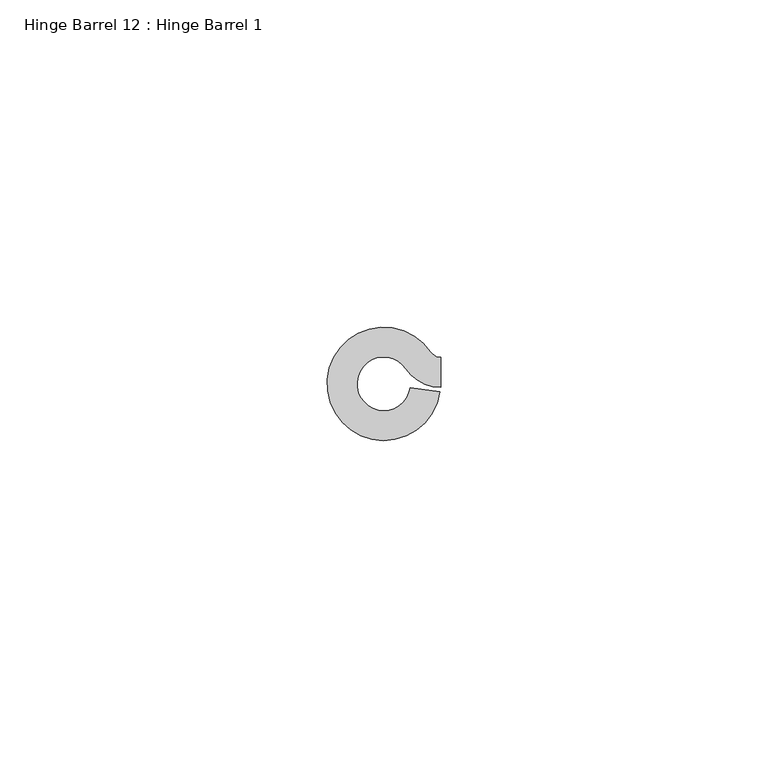
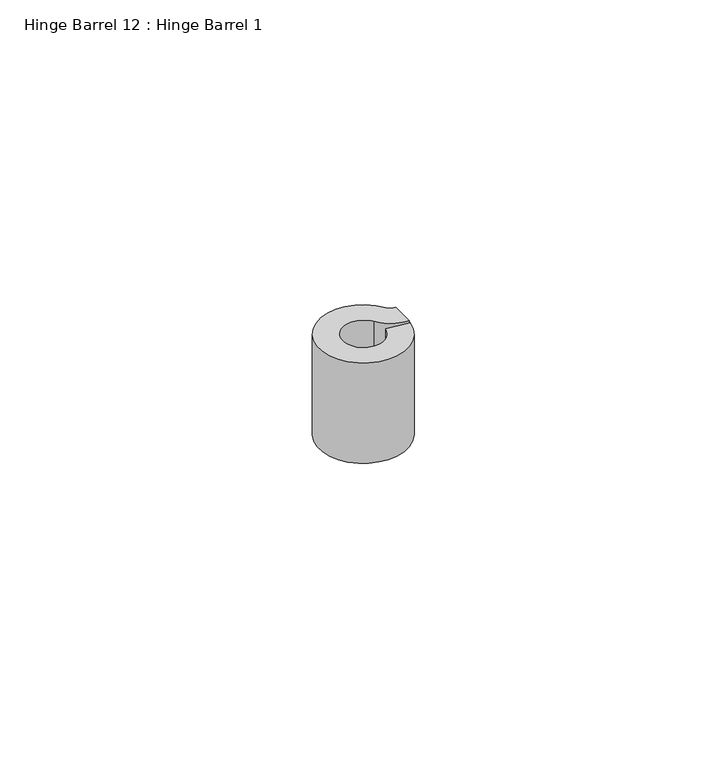
"""IFC4 building model written with IfcOpenShell, lengths in millimetres: proxy geometry, Hinge Barrel 12 : Hinge Barrel 1."""

import ifcopenshell
import ifcopenshell.guid

model = None  # the IFC model being written
_history = None  # IfcOwnerHistory: only IFC2X3 demands one
_inside = {}  # id of a spatial element -> (the spatial element, [elements in it])
_under = {}  # id of a project, library or spatial element -> (it, [spatial elements below it])
_declared = {}  # id of a project -> (the project, [libraries it declares])
_typed = {}  # id of a type object -> (the type object, [elements of that type])
_made_of = {}  # id of a material, layer set ... -> (it, [elements and type objects made of it])


def new_model(schema):
    """Start an empty IFC model of exactly this schema.

    Asked for "IFC4X3", IfcOpenShell would pick the latest addendum, in which some entities
    have other attributes; the version numbers below select the first issue.
    IFC2X3 requires an IfcOwnerHistory on every rooted entity: one is made here for all.
    """
    global model, _history
    if schema == "IFC4X3":
        model = ifcopenshell.file(schema_version=(4, 3, 0, 0))
    else:
        model = ifcopenshell.file(schema=schema)
    _inside.clear()
    _under.clear()
    _declared.clear()
    _typed.clear()
    _made_of.clear()
    _history = None
    if model.schema == "IFC2X3":
        org = make("IfcOrganization", Name="unknown")
        user = make(
            "IfcPersonAndOrganization",
            ThePerson=make("IfcPerson", FamilyName="unknown"),
            TheOrganization=org,
        )
        app = make(
            "IfcApplication",
            ApplicationDeveloper=org,
            Version="unknown",
            ApplicationFullName="unknown",
            ApplicationIdentifier="unknown",
        )
        _history = make(
            "IfcOwnerHistory",
            OwningUser=user,
            OwningApplication=app,
            ChangeAction="ADDED",
            CreationDate=0,
        )
    return model


def make(cls, **values):
    """One entity of the class cls with the attributes given. An attribute that is None is left unset."""
    return model.create_entity(
        cls, **{name: value for name, value in values.items() if value is not None}
    )


def rooted(cls, **values):
    """An entity with a GlobalId (a new one), such as an element, a storey or a relation."""
    return make(cls, GlobalId=ifcopenshell.guid.new(), OwnerHistory=_history, **values)


def si_unit(unit_type, name, prefix=None):
    """IfcSIUnit, for example si_unit("LENGTHUNIT", "METRE", prefix="MILLI")."""
    return make("IfcSIUnit", UnitType=unit_type, Prefix=prefix, Name=name)


def assignment(units):
    """IfcUnitAssignment: the units of a project."""
    return None if units is None else make("IfcUnitAssignment", Units=units)


def point(xyz):
    """IfcCartesianPoint."""
    return None if xyz is None else make("IfcCartesianPoint", Coordinates=xyz)


def direction(xyz):
    """IfcDirection."""
    return None if xyz is None else make("IfcDirection", DirectionRatios=xyz)


def frame(location, z_axis=None, x_axis=None):
    """IfcAxis2Placement3D, a coordinate frame: its origin and axes. An axis left out is left unset."""
    return make(
        "IfcAxis2Placement3D",
        Location=point(location),
        Axis=direction(z_axis),
        RefDirection=direction(x_axis),
    )


def frame_2d(location, x_axis=None):
    """IfcAxis2Placement2D, a coordinate frame in the plane: its origin and x axis."""
    return make(
        "IfcAxis2Placement2D", Location=point(location), RefDirection=direction(x_axis)
    )


def origin():
    """The frame at (0, 0, 0) with its axes left unset."""
    return frame((0.0, 0.0, 0.0))


def place(relative_to, where):
    """IfcLocalPlacement: puts the frame where relative to a parent placement (None: the world)."""
    return make(
        "IfcLocalPlacement", PlacementRelTo=relative_to, RelativePlacement=where
    )


def context(
    kind, dimensions, precision=None, world=None, true_north=None, identifier=None
):
    """IfcGeometricRepresentationContext, for example the 3D "Model" context."""
    return make(
        "IfcGeometricRepresentationContext",
        ContextIdentifier=identifier,
        ContextType=kind,
        CoordinateSpaceDimension=dimensions,
        Precision=precision,
        WorldCoordinateSystem=world,
        TrueNorth=true_north,
    )


def project(units=None, contexts=None):
    """IfcProject with its units and contexts."""
    return rooted(
        "IfcProject",
        Name="project",
        RepresentationContexts=contexts,
        UnitsInContext=assignment(units),
    )


def spatial(cls, under=None, at=None, **own):
    """A site, building, storey or space (cls), placed at a placement, below another one or the project."""
    s = rooted(cls, ObjectPlacement=at, **own)
    if under is not None:
        _under.setdefault(under.id(), (under, []))[1].append(s)
    return s


def polyline(points):
    """IfcPolyline through the points."""
    return make("IfcPolyline", Points=[point(p) for p in points])


def circle_curve(where, radius):
    """IfcCircle in the frame where."""
    return make("IfcCircle", Position=where, Radius=radius)


def trimmed(basis, trim1, trim2, sense, master):
    """IfcTrimmedCurve: the piece of a basis curve between two trims."""
    return make(
        "IfcTrimmedCurve",
        BasisCurve=basis,
        Trim1=trim1,
        Trim2=trim2,
        SenseAgreement=sense,
        MasterRepresentation=master,
    )


def segment(curve, same_sense, transition):
    """IfcCompositeCurveSegment."""
    return make(
        "IfcCompositeCurveSegment",
        Transition=transition,
        SameSense=same_sense,
        ParentCurve=curve,
    )


def composite_curve(segments, self_intersect=None):
    """IfcCompositeCurve: segments joined end to end."""
    return make("IfcCompositeCurve", Segments=segments, SelfIntersect=self_intersect)


def outline(outer, holes=None, kind="AREA"):
    """IfcArbitraryClosedProfileDef: a profile drawn as a closed curve; with holes, ...WithVoids."""
    if holes is None:
        return make("IfcArbitraryClosedProfileDef", ProfileType=kind, OuterCurve=outer)
    return make(
        "IfcArbitraryProfileDefWithVoids",
        ProfileType=kind,
        OuterCurve=outer,
        InnerCurves=holes,
    )


def extrude(swept, where, along, depth):
    """IfcExtrudedAreaSolid: the profile swept, set in the frame where, extruded along a direction by depth."""
    return make(
        "IfcExtrudedAreaSolid",
        SweptArea=swept,
        Position=where,
        ExtrudedDirection=direction(along),
        Depth=depth,
    )


def shape(context_of_items, identifier, shape_type, items):
    """IfcShapeRepresentation: the items that make up one representation, for example the "Body"."""
    return make(
        "IfcShapeRepresentation",
        ContextOfItems=context_of_items,
        RepresentationIdentifier=identifier,
        RepresentationType=shape_type,
        Items=items,
    )


def source(mapping_origin, context_of_items, identifier, shape_type, items):
    """IfcRepresentationMap: a shape defined once, which mapped items show again and again."""
    return make(
        "IfcRepresentationMap",
        MappingOrigin=mapping_origin,
        MappedRepresentation=shape(context_of_items, identifier, shape_type, items),
    )


def transform(
    local_origin,
    x_axis=None,
    y_axis=None,
    z_axis=None,
    scale=None,
    scale2=None,
    scale3=None,
    uniform=True,
):
    """IfcCartesianTransformationOperator3D, or its non-uniform kind. x_axis, y_axis, z_axis: its Axis1, 2, 3."""
    if uniform:
        return make(
            "IfcCartesianTransformationOperator3D",
            Axis1=direction(x_axis),
            Axis2=direction(y_axis),
            LocalOrigin=point(local_origin),
            Scale=scale,
            Axis3=direction(z_axis),
        )
    return make(
        "IfcCartesianTransformationOperator3DnonUniform",
        Axis1=direction(x_axis),
        Axis2=direction(y_axis),
        LocalOrigin=point(local_origin),
        Scale=scale,
        Axis3=direction(z_axis),
        Scale2=scale2,
        Scale3=scale3,
    )


def mapped(mapping_source, mapping_target):
    """IfcMappedItem: shows the shape of a source again, moved by a transform."""
    return make(
        "IfcMappedItem", MappingSource=mapping_source, MappingTarget=mapping_target
    )


def made_of(thing, what):
    """Note that an element or type object is made of a material, layer set ...; save() writes the relation."""
    if what is not None:
        _made_of.setdefault(what.id(), (what, []))[1].append(thing)
    return thing


def element(
    cls,
    number,
    at=None,
    inside=None,
    cuts=None,
    type_object=None,
    material=None,
    context=None,
    identifier="Body",
    shape_type=None,
    held_by="IfcProductDefinitionShape",
    body=None,
    shapes=None,
    **own,
):
    """One element of the class cls, such as IfcWall. Its Tag is "e" and its number.

    at: its placement. inside: the storey or other place that contains it. cuts: it is an
    opening in that element (IfcRelVoidsElement). A single representation is given by context,
    identifier, shape_type and body (its items); several are given by shapes. held_by: the class
    of the entity that holds the representations. save() writes the other relations.
    """
    e = rooted(cls, Tag="e%d" % number, ObjectPlacement=at, **own)
    if body is not None:
        shapes = [shape(context, identifier, shape_type, body)]
    if shapes is not None:
        e.Representation = make(held_by, Representations=shapes)
    if inside is not None:
        _inside.setdefault(inside.id(), (inside, []))[1].append(e)
    if cuts is not None:
        rooted(
            "IfcRelVoidsElement", RelatingBuildingElement=cuts, RelatedOpeningElement=e
        )
    if type_object is not None:
        _typed.setdefault(type_object.id(), (type_object, []))[1].append(e)
    return made_of(e, material)


def aggregate(whole, parts):
    """IfcRelAggregates: a whole, such as a stair, and the parts it consists of."""
    return rooted("IfcRelAggregates", RelatingObject=whole, RelatedObjects=parts)


def save(model, path):
    """Write the relations noted so far, then the file.

    IfcRelAggregates (storeys below a building ...), IfcRelContainedInSpatialStructure (elements
    in a storey), IfcRelDefinesByType, IfcRelAssociatesMaterial and IfcRelDeclares: one each for
    every whole, place, type object, material and project.
    """
    for whole, parts in _under.values():
        aggregate(whole, parts)
    for where, things in _inside.values():
        rooted(
            "IfcRelContainedInSpatialStructure",
            RelatedElements=things,
            RelatingStructure=where,
        )
    for kind, things in _typed.values():
        rooted("IfcRelDefinesByType", RelatedObjects=things, RelatingType=kind)
    for what, things in _made_of.values():
        rooted("IfcRelAssociatesMaterial", RelatedObjects=things, RelatingMaterial=what)
    for by, libraries in _declared.values():
        rooted("IfcRelDeclares", RelatingContext=by, RelatedDefinitions=libraries)
    model.write(path)


def hinge_barrel_12_hinge_barrel_1_babfa127(model_context):
    return source(origin(), model_context, "Body", "SweptSolid", [
        extrude(outline(composite_curve([segment(trimmed(circle_curve(frame_2d((587319.1320739, -531776.6049841)), 4.0894), [point((587322.5194669, -531774.3139665))], [point((587323.1821338, -531777.1708529))], True, "CARTESIAN"), True, "CONTINUOUS"), segment(polyline([(587323.1821338, -531777.1708529), (587327.7022899, -531777.8024028)]), True, "CONTINUOUS"), segment(trimmed(circle_curve(frame_2d((587319.1320739, -531776.6049841)), 8.6534625), [point((587327.7022899, -531777.8024028))], [point((587326.3000393, -531771.7570273))], False, "CARTESIAN"), True, "CONTINUOUS"), segment(trimmed(circle_curve(frame_2d((587327.8245257, -531770.7259615)), 1.8404226), [point((587326.3000393, -531771.7570273))], [point((587327.8245257, -531772.5663841))], True, "CARTESIAN"), True, "CONTINUOUS"), segment(polyline([(587327.8245257, -531772.5663841), (587327.8245257, -531777.1304466)]), True, "CONTINUOUS"), segment(trimmed(circle_curve(frame_2d((587327.8245257, -531770.7259615)), 6.4044851), [point((587327.8245257, -531777.1304466))], [point((587322.5194669, -531774.3139665))], False, "CARTESIAN"), True, "CONTINUOUS")], self_intersect=False)), frame((0.0, 0.0, 2063.75), z_axis=(0.0, 0.0, 1.0), x_axis=(1.0, 0.0, 0.0)), (0.0, 0.0, 1.0), 20.8359375),
    ])


if __name__ == "__main__":
    model = new_model("IFC4")
    model_context = context("Model", 3, world=origin())
    ifc_project = project(units=[si_unit("LENGTHUNIT", "METRE", prefix="MILLI")], contexts=[model_context])
    site = spatial("IfcSite", under=ifc_project)
    building = spatial("IfcBuilding", under=site)
    placement = place(None, origin())
    hinge_barrel_12_hinge_barrel_1_shape = hinge_barrel_12_hinge_barrel_1_babfa127(model_context)
    element("IfcBuildingElementProxy", 1, Name="Hinge Barrel 12 : Hinge Barrel 1", ObjectType="Hinge Barrel 12 : Hinge Barrel 1", at=placement, inside=building, context=model_context, shape_type="MappedRepresentation", body=[
        mapped(hinge_barrel_12_hinge_barrel_1_shape, transform((0.0, 0.0, 0.0), x_axis=(1.0, 0.0, 0.0), y_axis=(0.0, 1.0, 0.0), z_axis=(0.0, 0.0, 1.0))),
    ])
    save(model, "model.ifc")

# Revit data of these elements
# Element 1 (IfcBuildingElementProxy, "Hinge Barrel 12 : Hinge Barrel 1")
#   Materials on its faces: "6\"X6\" WELD-ON STL BUTT HINGE"
# Materials
#   "6\"X6\" WELD-ON STL BUTT HINGE": class "Metal", colour RGB 189 187 185, transparency 0, Description = "Carbon steel", Cost = 0
